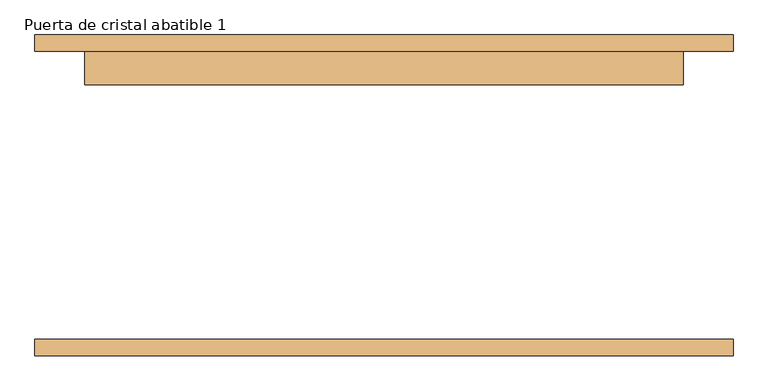
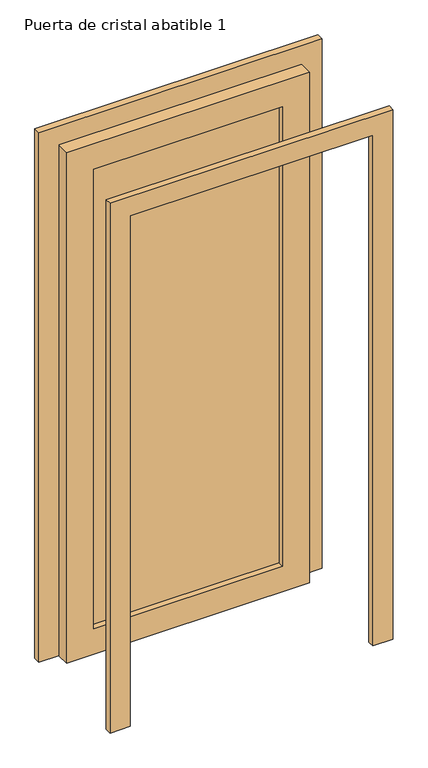
"""IFC4 building model written with IfcOpenShell, lengths in millimetres: door geometry, Puerta de cristal abatible 1 : PUERTA VIDRIO PABLO."""

from ifc_helpers import new_model, si_unit, frame, origin, place, context, project, spatial, polyline, outline, extrude, source, transform, mapped, element, save


def puerta_de_cristal_abatible_1_b968bd6e(model_context):
    return source(origin(), model_context, "Body", "SweptSolid", [
        extrude(outline(polyline([(2032.0, 457.5), (0.0, 457.5), (0.0, 533.5), (2108.0, 533.5), (2108.0, -533.5), (0.0, -533.5), (0.0, -457.5), (2032.0, -457.5), (2032.0, 457.5)])), frame((0.0, -245.0, 0.0), z_axis=(0.0, 1.0, 0.0), x_axis=(0.0, 0.0, 1.0)), (0.0, 0.0, 1.0), 25.0),
        extrude(outline(polyline([(2032.0, 457.5), (0.0, 457.5), (0.0, 533.5), (2108.0, 533.5), (2108.0, -533.5), (0.0, -533.5), (0.0, -457.5), (2032.0, -457.5), (2032.0, 457.5)])), frame((0.0, 220.0, 0.0), z_axis=(0.0, 1.0, 0.0), x_axis=(0.0, 0.0, 1.0)), (0.0, 0.0, 1.0), 25.0),
        extrude(outline(polyline([(355.5, 191.425), (-355.5, 191.425), (-355.5, 197.775), (355.5, 197.775), (355.5, 191.425)])), frame((0.0, 0.0, 102.0), z_axis=(0.0, 0.0, 1.0), x_axis=(1.0, 0.0, 0.0)), (0.0, 0.0, 1.0), 1828.0),
        extrude(outline(polyline([(2032.0, 457.5), (2032.0, -457.5), (0.0, -457.5), (0.0, 457.5), (2032.0, 457.5)]), holes=[polyline([(1930.0, -355.5), (1930.0, 355.5), (102.0, 355.5), (102.0, -355.5), (1930.0, -355.5)])]), frame((0.0, 169.0, 0.0), z_axis=(0.0, 1.0, 0.0), x_axis=(0.0, 0.0, 1.0)), (0.0, 0.0, 1.0), 51.0),
    ])


if __name__ == "__main__":
    model = new_model("IFC4")
    model_context = context("Model", 3, world=origin())
    ifc_project = project(units=[si_unit("LENGTHUNIT", "METRE", prefix="MILLI")], contexts=[model_context])
    site = spatial("IfcSite", under=ifc_project)
    building = spatial("IfcBuilding", under=site)
    placement = place(None, origin())
    puerta_de_cristal_abatible_1_shape = puerta_de_cristal_abatible_1_b968bd6e(model_context)
    element("IfcDoor", 1, ObjectType="Puerta de cristal abatible 1 : PUERTA VIDRIO PABLO", at=placement, inside=building, context=model_context, shape_type="MappedRepresentation", body=[
        mapped(puerta_de_cristal_abatible_1_shape, transform((0.0, 0.0, 0.0), x_axis=(1.0, 0.0, 0.0), y_axis=(0.0, 1.0, 0.0), z_axis=(0.0, 0.0, 1.0))),
    ])
    save(model, "model.ifc")

# Revit data of these elements
# Type "Puerta de cristal abatible 1 : PUERTA VIDRIO PABLO"
#   Description = "Puerta vidrio 1 hoja abatible"
#   Type Mark = "P2"
#   Construction Type Id = "SGL"
#   Analytic Construction = "Ventanas grandes con acristalamiento simple"
#   Visual Light Transmittance = 0.9
#   Thickness = 0.051 m
#   Solar Heat Gain Coefficient = 0.86
#   Heat Transfer Coefficient (U) = 5.5617 W/(m²·K)
#   Height = 2.032 m
#   Anchura de barandal - Base = 0.102 m
#   Anchura de barandal - Parte superior = 0.102 m
#   Anchura de montante - Bisagra = 0.102 m
#   Anchura de montante - Pasador = 0.102 m
#   Proyección cubrejuntas ext = 0.025 m
#   Proyección cubrejuntas int = 0.025 m
#   Anchura de cubrejuntas = 0.076 m
#   Width = 0.915 m
#   Define Thermal Properties by = 1
#   Material de puerta = Puerta - Panel
#   Material de estructura = Puerta - Marco
#   Function = (empty or 0)
#   Wall Closure = (empty or 0)
# Element 1 (IfcDoor, "Puerta de cristal abatible 1 : PUERTA VIDRIO PABLO")
#   Materials on its faces: "Puerta - Marco", "Puerta - Panel", "Vidrio"
# Materials
#   "Puerta - Panel": class "Madera", colour RGB 210 159 95, transparency 0
#   "Puerta - Marco": class "Madera", colour RGB 118 70 51, transparency 0
#   "Vidrio": class "Vidrio", colour RGB 0 128 192, transparency 0.75, Description = "Vidrio de cal sodada", Cost = 0
